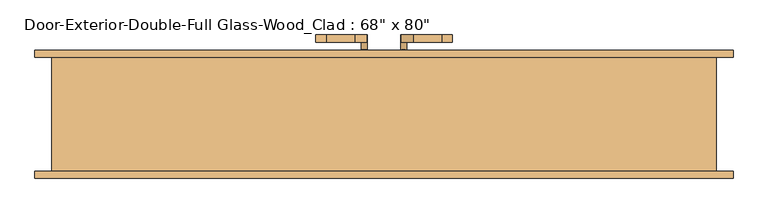
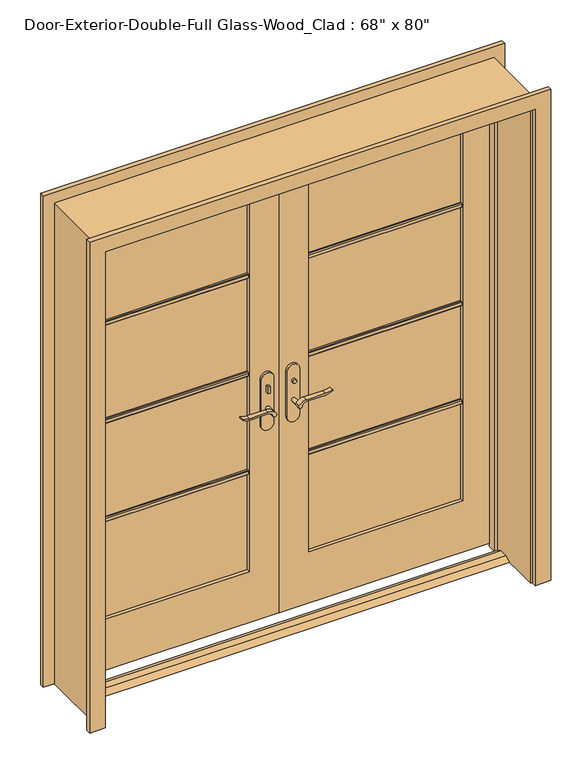
"""IFC4 building model written with IfcOpenShell, lengths in millimetres: door geometry."""

import ifcopenshell
import ifcopenshell.guid

model = None  # the IFC model being written
_history = None  # IfcOwnerHistory: only IFC2X3 demands one
_inside = {}  # id of a spatial element -> (the spatial element, [elements in it])
_under = {}  # id of a project, library or spatial element -> (it, [spatial elements below it])
_declared = {}  # id of a project -> (the project, [libraries it declares])
_typed = {}  # id of a type object -> (the type object, [elements of that type])
_made_of = {}  # id of a material, layer set ... -> (it, [elements and type objects made of it])


def new_model(schema):
    """Start an empty IFC model of exactly this schema.

    Asked for "IFC4X3", IfcOpenShell would pick the latest addendum, in which some entities
    have other attributes; the version numbers below select the first issue.
    IFC2X3 requires an IfcOwnerHistory on every rooted entity: one is made here for all.
    """
    global model, _history
    if schema == "IFC4X3":
        model = ifcopenshell.file(schema_version=(4, 3, 0, 0))
    else:
        model = ifcopenshell.file(schema=schema)
    _inside.clear()
    _under.clear()
    _declared.clear()
    _typed.clear()
    _made_of.clear()
    _history = None
    if model.schema == "IFC2X3":
        org = make("IfcOrganization", Name="unknown")
        user = make(
            "IfcPersonAndOrganization",
            ThePerson=make("IfcPerson", FamilyName="unknown"),
            TheOrganization=org,
        )
        app = make(
            "IfcApplication",
            ApplicationDeveloper=org,
            Version="unknown",
            ApplicationFullName="unknown",
            ApplicationIdentifier="unknown",
        )
        _history = make(
            "IfcOwnerHistory",
            OwningUser=user,
            OwningApplication=app,
            ChangeAction="ADDED",
            CreationDate=0,
        )
    return model


def make(cls, **values):
    """One entity of the class cls with the attributes given. An attribute that is None is left unset."""
    return model.create_entity(
        cls, **{name: value for name, value in values.items() if value is not None}
    )


def rooted(cls, **values):
    """An entity with a GlobalId (a new one), such as an element, a storey or a relation."""
    return make(cls, GlobalId=ifcopenshell.guid.new(), OwnerHistory=_history, **values)


def si_unit(unit_type, name, prefix=None):
    """IfcSIUnit, for example si_unit("LENGTHUNIT", "METRE", prefix="MILLI")."""
    return make("IfcSIUnit", UnitType=unit_type, Prefix=prefix, Name=name)


def assignment(units):
    """IfcUnitAssignment: the units of a project."""
    return None if units is None else make("IfcUnitAssignment", Units=units)


def point(xyz):
    """IfcCartesianPoint."""
    return None if xyz is None else make("IfcCartesianPoint", Coordinates=xyz)


def direction(xyz):
    """IfcDirection."""
    return None if xyz is None else make("IfcDirection", DirectionRatios=xyz)


def frame(location, z_axis=None, x_axis=None):
    """IfcAxis2Placement3D, a coordinate frame: its origin and axes. An axis left out is left unset."""
    return make(
        "IfcAxis2Placement3D",
        Location=point(location),
        Axis=direction(z_axis),
        RefDirection=direction(x_axis),
    )


def frame_2d(location, x_axis=None):
    """IfcAxis2Placement2D, a coordinate frame in the plane: its origin and x axis."""
    return make(
        "IfcAxis2Placement2D", Location=point(location), RefDirection=direction(x_axis)
    )


def origin():
    """The frame at (0, 0, 0) with its axes left unset."""
    return frame((0.0, 0.0, 0.0))


def place(relative_to, where):
    """IfcLocalPlacement: puts the frame where relative to a parent placement (None: the world)."""
    return make(
        "IfcLocalPlacement", PlacementRelTo=relative_to, RelativePlacement=where
    )


def context(
    kind, dimensions, precision=None, world=None, true_north=None, identifier=None
):
    """IfcGeometricRepresentationContext, for example the 3D "Model" context."""
    return make(
        "IfcGeometricRepresentationContext",
        ContextIdentifier=identifier,
        ContextType=kind,
        CoordinateSpaceDimension=dimensions,
        Precision=precision,
        WorldCoordinateSystem=world,
        TrueNorth=true_north,
    )


def project(units=None, contexts=None):
    """IfcProject with its units and contexts."""
    return rooted(
        "IfcProject",
        Name="project",
        RepresentationContexts=contexts,
        UnitsInContext=assignment(units),
    )


def spatial(cls, under=None, at=None, **own):
    """A site, building, storey or space (cls), placed at a placement, below another one or the project."""
    s = rooted(cls, ObjectPlacement=at, **own)
    if under is not None:
        _under.setdefault(under.id(), (under, []))[1].append(s)
    return s


def polyline(points):
    """IfcPolyline through the points."""
    return make("IfcPolyline", Points=[point(p) for p in points])


def circle_curve(where, radius):
    """IfcCircle in the frame where."""
    return make("IfcCircle", Position=where, Radius=radius)


def trimmed(basis, trim1, trim2, sense, master):
    """IfcTrimmedCurve: the piece of a basis curve between two trims."""
    return make(
        "IfcTrimmedCurve",
        BasisCurve=basis,
        Trim1=trim1,
        Trim2=trim2,
        SenseAgreement=sense,
        MasterRepresentation=master,
    )


def segment(curve, same_sense, transition):
    """IfcCompositeCurveSegment."""
    return make(
        "IfcCompositeCurveSegment",
        Transition=transition,
        SameSense=same_sense,
        ParentCurve=curve,
    )


def composite_curve(segments, self_intersect=None):
    """IfcCompositeCurve: segments joined end to end."""
    return make("IfcCompositeCurve", Segments=segments, SelfIntersect=self_intersect)


def outline(outer, holes=None, kind="AREA"):
    """IfcArbitraryClosedProfileDef: a profile drawn as a closed curve; with holes, ...WithVoids."""
    if holes is None:
        return make("IfcArbitraryClosedProfileDef", ProfileType=kind, OuterCurve=outer)
    return make(
        "IfcArbitraryProfileDefWithVoids",
        ProfileType=kind,
        OuterCurve=outer,
        InnerCurves=holes,
    )


def extrude(swept, where, along, depth):
    """IfcExtrudedAreaSolid: the profile swept, set in the frame where, extruded along a direction by depth."""
    return make(
        "IfcExtrudedAreaSolid",
        SweptArea=swept,
        Position=where,
        ExtrudedDirection=direction(along),
        Depth=depth,
    )


def faces_of(points, faces, orient=None, outer=None):
    """IfcFace entities. A face is a list of loops; a loop is a list of indices into points, from 0.

    orient and outer hold one flag for each loop. By default every Orientation is true, the
    first loop of a face is its IfcFaceOuterBound and the others are IfcFaceBound.
    """
    made = []
    for i, loops in enumerate(faces):
        bounds = []
        for j, loop in enumerate(loops):
            is_outer = j == 0 if outer is None else outer[i][j]
            bounds.append(
                make(
                    "IfcFaceOuterBound" if is_outer else "IfcFaceBound",
                    Bound=make("IfcPolyLoop", Polygon=[points[k] for k in loop]),
                    Orientation=True if orient is None else orient[i][j],
                )
            )
        made.append(make("IfcFace", Bounds=bounds))
    return made


def faceted_brep(points, faces, orient=None, outer=None, voids=None):
    """IfcFacetedBrep: a solid bounded by flat faces; with voids (closed shells), ...WithVoids."""
    shared = [point(p) for p in points]
    hull = make("IfcClosedShell", CfsFaces=faces_of(shared, faces, orient, outer))
    if voids is None:
        return make("IfcFacetedBrep", Outer=hull)
    return make(
        "IfcFacetedBrepWithVoids",
        Outer=hull,
        Voids=[
            make(cls, CfsFaces=faces_of(shared, fs, o, b)) for cls, fs, o, b in voids
        ],
    )


def shape(context_of_items, identifier, shape_type, items):
    """IfcShapeRepresentation: the items that make up one representation, for example the "Body"."""
    return make(
        "IfcShapeRepresentation",
        ContextOfItems=context_of_items,
        RepresentationIdentifier=identifier,
        RepresentationType=shape_type,
        Items=items,
    )


def source(mapping_origin, context_of_items, identifier, shape_type, items):
    """IfcRepresentationMap: a shape defined once, which mapped items show again and again."""
    return make(
        "IfcRepresentationMap",
        MappingOrigin=mapping_origin,
        MappedRepresentation=shape(context_of_items, identifier, shape_type, items),
    )


def transform(
    local_origin,
    x_axis=None,
    y_axis=None,
    z_axis=None,
    scale=None,
    scale2=None,
    scale3=None,
    uniform=True,
):
    """IfcCartesianTransformationOperator3D, or its non-uniform kind. x_axis, y_axis, z_axis: its Axis1, 2, 3."""
    if uniform:
        return make(
            "IfcCartesianTransformationOperator3D",
            Axis1=direction(x_axis),
            Axis2=direction(y_axis),
            LocalOrigin=point(local_origin),
            Scale=scale,
            Axis3=direction(z_axis),
        )
    return make(
        "IfcCartesianTransformationOperator3DnonUniform",
        Axis1=direction(x_axis),
        Axis2=direction(y_axis),
        LocalOrigin=point(local_origin),
        Scale=scale,
        Axis3=direction(z_axis),
        Scale2=scale2,
        Scale3=scale3,
    )


def mapped(mapping_source, mapping_target):
    """IfcMappedItem: shows the shape of a source again, moved by a transform."""
    return make(
        "IfcMappedItem", MappingSource=mapping_source, MappingTarget=mapping_target
    )


def made_of(thing, what):
    """Note that an element or type object is made of a material, layer set ...; save() writes the relation."""
    if what is not None:
        _made_of.setdefault(what.id(), (what, []))[1].append(thing)
    return thing


def element(
    cls,
    number,
    at=None,
    inside=None,
    cuts=None,
    type_object=None,
    material=None,
    context=None,
    identifier="Body",
    shape_type=None,
    held_by="IfcProductDefinitionShape",
    body=None,
    shapes=None,
    **own,
):
    """One element of the class cls, such as IfcWall. Its Tag is "e" and its number.

    at: its placement. inside: the storey or other place that contains it. cuts: it is an
    opening in that element (IfcRelVoidsElement). A single representation is given by context,
    identifier, shape_type and body (its items); several are given by shapes. held_by: the class
    of the entity that holds the representations. save() writes the other relations.
    """
    e = rooted(cls, Tag="e%d" % number, ObjectPlacement=at, **own)
    if body is not None:
        shapes = [shape(context, identifier, shape_type, body)]
    if shapes is not None:
        e.Representation = make(held_by, Representations=shapes)
    if inside is not None:
        _inside.setdefault(inside.id(), (inside, []))[1].append(e)
    if cuts is not None:
        rooted(
            "IfcRelVoidsElement", RelatingBuildingElement=cuts, RelatedOpeningElement=e
        )
    if type_object is not None:
        _typed.setdefault(type_object.id(), (type_object, []))[1].append(e)
    return made_of(e, material)


def aggregate(whole, parts):
    """IfcRelAggregates: a whole, such as a stair, and the parts it consists of."""
    return rooted("IfcRelAggregates", RelatingObject=whole, RelatedObjects=parts)


def save(model, path):
    """Write the relations noted so far, then the file.

    IfcRelAggregates (storeys below a building ...), IfcRelContainedInSpatialStructure (elements
    in a storey), IfcRelDefinesByType, IfcRelAssociatesMaterial and IfcRelDeclares: one each for
    every whole, place, type object, material and project.
    """
    for whole, parts in _under.values():
        aggregate(whole, parts)
    for where, things in _inside.values():
        rooted(
            "IfcRelContainedInSpatialStructure",
            RelatedElements=things,
            RelatingStructure=where,
        )
    for kind, things in _typed.values():
        rooted("IfcRelDefinesByType", RelatedObjects=things, RelatingType=kind)
    for what, things in _made_of.values():
        rooted("IfcRelAssociatesMaterial", RelatedObjects=things, RelatingMaterial=what)
    for by, libraries in _declared.values():
        rooted("IfcRelDeclares", RelatingContext=by, RelatedDefinitions=libraries)
    model.write(path)


def door_f3362da7(model_context):
    return source(origin(), model_context, "Body", "SolidModel", [
        extrude(outline(polyline([(19.05, 12.7), (53.975, 12.7), (79.375, 0.0), (-6.35, 0.0), (19.05, 12.7)])), frame((-863.6, 0.0, 0.0), z_axis=(1.0, 0.0, 0.0), x_axis=(0.0, 1.0, 0.0)), (0.0, 0.0, 1.0), 1727.2),
        extrude(outline(polyline([(-47.4019111, 94.3), (-57.4019111, 94.3), (-57.4019111, 104.3), (-47.4019111, 104.3), (-47.4019111, 94.3)])), frame((0.0, 0.0, 981.9), z_axis=(0.0, 0.0, 1.0), x_axis=(1.0, 0.0, 0.0)), (0.0, 0.0, 1.0), 30.0),
        extrude(outline(composite_curve([segment(trimmed(circle_curve(frame_2d((996.9, -52.4019111)), 8.0), [point((996.9, -60.4019111))], [point((996.9, -44.4019111))], False, "CARTESIAN"), True, "CONTINUOUS"), segment(trimmed(circle_curve(frame_2d((996.9, -52.4019111)), 8.0), [point((996.9, -44.4019111))], [point((996.9, -60.4019111))], False, "CARTESIAN"), True, "CONTINUOUS")], self_intersect=False)), frame((0.0, 159.225, 0.0), z_axis=(0.0, 1.0, 0.0), x_axis=(0.0, 0.0, 1.0)), (0.0, 0.0, 1.0), 10.0),
        extrude(outline(composite_curve([segment(trimmed(circle_curve(frame_2d((897.1555521, -76.0694241)), 37.2832219), [point((919.0523287, -45.8937749))], [point((934.4, -77.7693445))], False, "CARTESIAN"), True, "CONTINUOUS"), segment(polyline([(934.4, -77.7693445), (934.4, -154.045502)]), True, "CONTINUOUS"), segment(trimmed(circle_curve(frame_2d((1017.6850638, -153.9791202)), 83.2850902), [point((934.4, -154.045502))], [point((939.4, -182.4019111))], True, "CARTESIAN"), True, "CONTINUOUS"), segment(polyline([(939.4, -182.4019111), (936.6135558, -182.4019111)]), True, "CONTINUOUS"), segment(trimmed(circle_curve(frame_2d((986.6709207, -150.4622499)), 59.3791355), [point((936.6135558, -182.4019111))], [point((927.4, -154.045502))], False, "CARTESIAN"), True, "CONTINUOUS"), segment(polyline([(927.4, -154.045502), (927.4, -77.7881013)]), True, "CONTINUOUS"), segment(trimmed(circle_curve(frame_2d((909.2738613, -77.7881013)), 18.1261387), [point((927.4, -77.7881013))], [point((914.4, -60.4019111))], True, "CARTESIAN"), True, "CONTINUOUS"), segment(trimmed(circle_curve(frame_2d((914.4, -52.4019111)), 8.0), [point((914.4, -60.4019111))], [point((919.0523287, -45.8937749))], False, "CARTESIAN"), True, "CONTINUOUS")], self_intersect=False)), frame((0.0, 54.3, 0.0), z_axis=(0.0, 1.0, 0.0), x_axis=(0.0, 0.0, 1.0)), (0.0, 0.0, 1.0), 20.0),
        extrude(outline(composite_curve([segment(trimmed(circle_curve(frame_2d((914.4, -52.4019111)), 8.0), [point((914.3999903, -60.4019111))], [point((919.0523287, -45.8937749))], False, "CARTESIAN"), True, "CONTINUOUS"), segment(trimmed(circle_curve(frame_2d((897.1555521, -76.0694241)), 37.2832219), [point((919.0523287, -45.8937749))], [point((934.4, -77.7693445))], False, "CARTESIAN"), True, "CONTINUOUS"), segment(polyline([(934.4, -77.7693445), (934.4, -154.045502)]), True, "CONTINUOUS"), segment(trimmed(circle_curve(frame_2d((1017.6850638, -153.9791202)), 83.2850902), [point((934.4, -154.045502))], [point((939.4, -182.4019111))], True, "CARTESIAN"), True, "CONTINUOUS"), segment(polyline([(939.4, -182.4019111), (936.6135558, -182.4019111)]), True, "CONTINUOUS"), segment(trimmed(circle_curve(frame_2d((986.6709207, -150.4622499)), 59.3791355), [point((936.6135558, -182.4019111))], [point((927.4, -154.045502))], False, "CARTESIAN"), True, "CONTINUOUS"), segment(polyline([(927.4, -154.045502), (927.4, -77.788099)]), True, "CONTINUOUS"), segment(trimmed(circle_curve(frame_2d((909.2738682, -77.788099)), 18.1261318), [point((927.4, -77.788099))], [point((914.3999903, -60.4019111))], True, "CARTESIAN"), True, "CONTINUOUS")], self_intersect=False)), frame((0.0, 189.225, 0.0), z_axis=(0.0, 1.0, 0.0), x_axis=(0.0, 0.0, 1.0)), (0.0, 0.0, 1.0), 20.0),
        extrude(outline(composite_curve([segment(trimmed(circle_curve(frame_2d((914.4, -52.4019111)), 8.0), [point((914.4, -60.4019111))], [point((914.4, -44.4019111))], False, "CARTESIAN"), True, "CONTINUOUS"), segment(trimmed(circle_curve(frame_2d((914.4, -52.4019111)), 8.0), [point((914.4, -44.4019111))], [point((914.4, -60.4019111))], False, "CARTESIAN"), True, "CONTINUOUS")], self_intersect=False)), frame((0.0, 74.3, 0.0), z_axis=(0.0, 1.0, 0.0), x_axis=(0.0, 0.0, 1.0)), (0.0, 0.0, 1.0), 30.0),
        extrude(outline(composite_curve([segment(trimmed(circle_curve(frame_2d((914.4, -52.4019111)), 8.0), [point((914.4, -60.4019111))], [point((914.4, -44.4019111))], False, "CARTESIAN"), True, "CONTINUOUS"), segment(trimmed(circle_curve(frame_2d((914.4, -52.4019111)), 8.0), [point((914.4, -44.4019111))], [point((914.4, -60.4019111))], False, "CARTESIAN"), True, "CONTINUOUS")], self_intersect=False)), frame((0.0, 159.225, 0.0), z_axis=(0.0, 1.0, 0.0), x_axis=(0.0, 0.0, 1.0)), (0.0, 0.0, 1.0), 30.0),
        extrude(outline(composite_curve([segment(polyline([(844.4, -27.4019111), (1039.4, -27.4019111)]), True, "CONTINUOUS"), segment(trimmed(circle_curve(frame_2d((1039.4, -52.4019111)), 25.0), [point((1039.4, -27.4019111))], [point((1039.4, -77.4019111))], False, "CARTESIAN"), True, "CONTINUOUS"), segment(polyline([(1039.4, -77.4019111), (844.4, -77.4019111)]), True, "CONTINUOUS"), segment(trimmed(circle_curve(frame_2d((844.4, -52.4019111)), 25.0), [point((844.4, -77.4019111))], [point((844.4, -27.4019111))], False, "CARTESIAN"), True, "CONTINUOUS")], self_intersect=False)), frame((0.0, 104.3, 0.0), z_axis=(0.0, 1.0, 0.0), x_axis=(0.0, 0.0, 1.0)), (0.0, 0.0, 1.0), 10.0),
        extrude(outline(composite_curve([segment(polyline([(844.4, -27.4019111), (1039.4, -27.4019111)]), True, "CONTINUOUS"), segment(trimmed(circle_curve(frame_2d((1039.4, -52.4019111)), 25.0), [point((1039.4, -27.4019111))], [point((1039.4, -77.4019111))], False, "CARTESIAN"), True, "CONTINUOUS"), segment(polyline([(1039.4, -77.4019111), (844.4, -77.4019111)]), True, "CONTINUOUS"), segment(trimmed(circle_curve(frame_2d((844.4, -52.4019111)), 25.0), [point((844.4, -77.4019111))], [point((844.4, -27.4019111))], False, "CARTESIAN"), True, "CONTINUOUS")], self_intersect=False)), frame((0.0, 149.225, 0.0), z_axis=(0.0, 1.0, 0.0), x_axis=(0.0, 0.0, 1.0)), (0.0, 0.0, 1.0), 10.0),
        extrude(outline(polyline([(47.3875, 169.225), (57.3875, 169.225), (57.3875, 159.225), (47.3875, 159.225), (47.3875, 169.225)])), frame((0.0, 0.0, 981.9), z_axis=(0.0, 0.0, 1.0), x_axis=(1.0, 0.0, 0.0)), (0.0, 0.0, 1.0), 30.0),
        extrude(outline(composite_curve([segment(trimmed(circle_curve(frame_2d((996.9, 52.3875)), 8.0), [point((996.9, 60.3875))], [point((996.9, 44.3875))], False, "CARTESIAN"), True, "CONTINUOUS"), segment(trimmed(circle_curve(frame_2d((996.9, 52.3875)), 8.0), [point((996.9, 44.3875))], [point((996.9, 60.3875))], False, "CARTESIAN"), True, "CONTINUOUS")], self_intersect=False)), frame((0.0, 94.3, 0.0), z_axis=(0.0, 1.0, 0.0), x_axis=(0.0, 0.0, 1.0)), (0.0, 0.0, 1.0), 10.0),
        extrude(outline(composite_curve([segment(trimmed(circle_curve(frame_2d((914.4, 52.3875)), 8.0), [point((919.0523287, 45.8793637))], [point((914.4, 60.3875))], False, "CARTESIAN"), True, "CONTINUOUS"), segment(trimmed(circle_curve(frame_2d((909.2738613, 77.7736901)), 18.1261387), [point((914.4, 60.3875))], [point((927.4, 77.7736901))], True, "CARTESIAN"), True, "CONTINUOUS"), segment(polyline([(927.4, 77.7736901), (927.4, 154.0310909)]), True, "CONTINUOUS"), segment(trimmed(circle_curve(frame_2d((986.6709207, 150.4478388)), 59.3791355), [point((927.4, 154.0310909))], [point((936.6135558, 182.3875))], False, "CARTESIAN"), True, "CONTINUOUS"), segment(polyline([(936.6135558, 182.3875), (939.4, 182.3875)]), True, "CONTINUOUS"), segment(trimmed(circle_curve(frame_2d((1017.6850638, 153.9647091)), 83.2850902), [point((939.4, 182.3875))], [point((934.4, 154.0310909))], True, "CARTESIAN"), True, "CONTINUOUS"), segment(polyline([(934.4, 154.0310909), (934.4, 77.7549333)]), True, "CONTINUOUS"), segment(trimmed(circle_curve(frame_2d((897.1555521, 76.0550129)), 37.2832219), [point((934.4, 77.7549333))], [point((919.0523287, 45.8793637))], False, "CARTESIAN"), True, "CONTINUOUS")], self_intersect=False)), frame((0.0, 189.225, 0.0), z_axis=(0.0, 1.0, 0.0), x_axis=(0.0, 0.0, 1.0)), (0.0, 0.0, 1.0), 20.0),
        extrude(outline(composite_curve([segment(trimmed(circle_curve(frame_2d((909.2738682, 77.7736878)), 18.1261318), [point((914.3999903, 60.3875))], [point((927.4, 77.7736878))], True, "CARTESIAN"), True, "CONTINUOUS"), segment(polyline([(927.4, 77.7736878), (927.4, 154.0310909)]), True, "CONTINUOUS"), segment(trimmed(circle_curve(frame_2d((986.6709207, 150.4478388)), 59.3791355), [point((927.4, 154.0310909))], [point((936.6135558, 182.3875))], False, "CARTESIAN"), True, "CONTINUOUS"), segment(polyline([(936.6135558, 182.3875), (939.4, 182.3875)]), True, "CONTINUOUS"), segment(trimmed(circle_curve(frame_2d((1017.6850638, 153.9647091)), 83.2850902), [point((939.4, 182.3875))], [point((934.4, 154.0310909))], True, "CARTESIAN"), True, "CONTINUOUS"), segment(polyline([(934.4, 154.0310909), (934.4, 77.7549333)]), True, "CONTINUOUS"), segment(trimmed(circle_curve(frame_2d((897.1555521, 76.0550129)), 37.2832219), [point((934.4, 77.7549333))], [point((919.0523287, 45.8793637))], False, "CARTESIAN"), True, "CONTINUOUS"), segment(trimmed(circle_curve(frame_2d((914.4, 52.3875)), 8.0), [point((919.0523287, 45.8793637))], [point((914.3999903, 60.3875))], False, "CARTESIAN"), True, "CONTINUOUS")], self_intersect=False)), frame((0.0, 54.3, 0.0), z_axis=(0.0, 1.0, 0.0), x_axis=(0.0, 0.0, 1.0)), (0.0, 0.0, 1.0), 20.0),
        extrude(outline(composite_curve([segment(trimmed(circle_curve(frame_2d((914.4, 52.3875)), 8.0), [point((914.4, 60.3875))], [point((914.4, 44.3875))], False, "CARTESIAN"), True, "CONTINUOUS"), segment(trimmed(circle_curve(frame_2d((914.4, 52.3875)), 8.0), [point((914.4, 44.3875))], [point((914.4, 60.3875))], False, "CARTESIAN"), True, "CONTINUOUS")], self_intersect=False)), frame((0.0, 159.225, 0.0), z_axis=(0.0, 1.0, 0.0), x_axis=(0.0, 0.0, 1.0)), (0.0, 0.0, 1.0), 30.0),
        extrude(outline(composite_curve([segment(trimmed(circle_curve(frame_2d((914.4, 52.3875)), 8.0), [point((914.4, 60.3875))], [point((914.4, 44.3875))], False, "CARTESIAN"), True, "CONTINUOUS"), segment(trimmed(circle_curve(frame_2d((914.4, 52.3875)), 8.0), [point((914.4, 44.3875))], [point((914.4, 60.3875))], False, "CARTESIAN"), True, "CONTINUOUS")], self_intersect=False)), frame((0.0, 74.3, 0.0), z_axis=(0.0, 1.0, 0.0), x_axis=(0.0, 0.0, 1.0)), (0.0, 0.0, 1.0), 30.0),
        extrude(outline(composite_curve([segment(trimmed(circle_curve(frame_2d((844.4, 52.3875)), 25.0), [point((844.4, 27.3875))], [point((844.4, 77.3875))], False, "CARTESIAN"), True, "CONTINUOUS"), segment(polyline([(844.4, 77.3875), (1039.4, 77.3875)]), True, "CONTINUOUS"), segment(trimmed(circle_curve(frame_2d((1039.4, 52.3875)), 25.0), [point((1039.4, 77.3875))], [point((1039.4, 27.3875))], False, "CARTESIAN"), True, "CONTINUOUS"), segment(polyline([(1039.4, 27.3875), (844.4, 27.3875)]), True, "CONTINUOUS")], self_intersect=False)), frame((0.0, 149.225, 0.0), z_axis=(0.0, 1.0, 0.0), x_axis=(0.0, 0.0, 1.0)), (0.0, 0.0, 1.0), 10.0),
        extrude(outline(composite_curve([segment(trimmed(circle_curve(frame_2d((844.4, 52.3875)), 25.0), [point((844.4, 27.3875))], [point((844.4, 77.3875))], False, "CARTESIAN"), True, "CONTINUOUS"), segment(polyline([(844.4, 77.3875), (1039.4, 77.3875)]), True, "CONTINUOUS"), segment(trimmed(circle_curve(frame_2d((1039.4, 52.3875)), 25.0), [point((1039.4, 77.3875))], [point((1039.4, 27.3875))], False, "CARTESIAN"), True, "CONTINUOUS"), segment(polyline([(1039.4, 27.3875), (844.4, 27.3875)]), True, "CONTINUOUS")], self_intersect=False)), frame((0.0, 104.3, 0.0), z_axis=(0.0, 1.0, 0.0), x_axis=(0.0, 0.0, 1.0)), (0.0, 0.0, 1.0), 10.0),
        extrude(outline(polyline([(128.27, 1502.171875), (128.27, 1483.121875), (121.92, 1483.121875), (118.745, 1486.296875), (118.745, 1498.996875), (121.92, 1502.171875), (128.27, 1502.171875)])), frame((120.65, 0.0, 0.0), z_axis=(1.0, 0.0, 0.0), x_axis=(0.0, 1.0, 0.0)), (0.0, 0.0, 1.0), 622.3),
        extrude(outline(polyline([(128.27, 1081.88125), (128.27, 1062.83125), (121.92, 1062.83125), (118.745, 1066.00625), (118.745, 1078.70625), (121.92, 1081.88125), (128.27, 1081.88125)])), frame((120.65, 0.0, 0.0), z_axis=(1.0, 0.0, 0.0), x_axis=(0.0, 1.0, 0.0)), (0.0, 0.0, 1.0), 622.3),
        extrude(outline(polyline([(128.27, 661.590625), (128.27, 642.540625), (121.92, 642.540625), (118.745, 645.715625), (118.745, 658.415625), (121.92, 661.590625), (128.27, 661.590625)])), frame((120.65, 0.0, 0.0), z_axis=(1.0, 0.0, 0.0), x_axis=(0.0, 1.0, 0.0)), (0.0, 0.0, 1.0), 622.3),
        extrude(outline(polyline([(135.255, 1502.171875), (141.605, 1502.171875), (144.78, 1498.996875), (144.78, 1486.296875), (141.605, 1483.121875), (135.255, 1483.121875), (135.255, 1502.171875)])), frame((-742.95, 0.0, 0.0), z_axis=(1.0, 0.0, 0.0), x_axis=(0.0, 1.0, 0.0)), (0.0, 0.0, 1.0), 622.3),
        extrude(outline(polyline([(135.255, 1081.88125), (141.605, 1081.88125), (144.78, 1078.70625), (144.78, 1066.00625), (141.605, 1062.83125), (135.255, 1062.83125), (135.255, 1081.88125)])), frame((-742.95, 0.0, 0.0), z_axis=(1.0, 0.0, 0.0), x_axis=(0.0, 1.0, 0.0)), (0.0, 0.0, 1.0), 622.3),
        extrude(outline(polyline([(135.255, 661.590625), (141.605, 661.590625), (144.78, 658.415625), (144.78, 645.715625), (141.605, 642.540625), (135.255, 642.540625), (135.255, 661.590625)])), frame((-742.95, 0.0, 0.0), z_axis=(1.0, 0.0, 0.0), x_axis=(0.0, 1.0, 0.0)), (0.0, 0.0, 1.0), 622.3),
        extrude(outline(polyline([(135.255, 1502.171875), (141.605, 1502.171875), (144.78, 1498.996875), (144.78, 1486.296875), (141.605, 1483.121875), (135.255, 1483.121875), (135.255, 1502.171875)])), frame((120.65, 0.0, 0.0), z_axis=(1.0, 0.0, 0.0), x_axis=(0.0, 1.0, 0.0)), (0.0, 0.0, 1.0), 622.3),
        extrude(outline(polyline([(135.255, 1081.88125), (141.605, 1081.88125), (144.78, 1078.70625), (144.78, 1066.00625), (141.605, 1062.83125), (135.255, 1062.83125), (135.255, 1081.88125)])), frame((120.65, 0.0, 0.0), z_axis=(1.0, 0.0, 0.0), x_axis=(0.0, 1.0, 0.0)), (0.0, 0.0, 1.0), 622.3),
        extrude(outline(polyline([(135.255, 661.590625), (141.605, 661.590625), (144.78, 658.415625), (144.78, 645.715625), (141.605, 642.540625), (135.255, 642.540625), (135.255, 661.590625)])), frame((120.65, 0.0, 0.0), z_axis=(1.0, 0.0, 0.0), x_axis=(0.0, 1.0, 0.0)), (0.0, 0.0, 1.0), 622.3),
        extrude(outline(polyline([(128.27, 1502.171875), (128.27, 1483.121875), (121.92, 1483.121875), (118.745, 1486.296875), (118.745, 1498.996875), (121.92, 1502.171875), (128.27, 1502.171875)])), frame((-742.95, 0.0, 0.0), z_axis=(1.0, 0.0, 0.0), x_axis=(0.0, 1.0, 0.0)), (0.0, 0.0, 1.0), 622.3),
        extrude(outline(polyline([(128.27, 1081.88125), (128.27, 1062.83125), (121.92, 1062.83125), (118.745, 1066.00625), (118.745, 1078.70625), (121.92, 1081.88125), (128.27, 1081.88125)])), frame((-742.95, 0.0, 0.0), z_axis=(1.0, 0.0, 0.0), x_axis=(0.0, 1.0, 0.0)), (0.0, 0.0, 1.0), 622.3),
        extrude(outline(polyline([(128.27, 661.590625), (128.27, 642.540625), (121.92, 642.540625), (118.745, 645.715625), (118.745, 658.415625), (121.92, 661.590625), (128.27, 661.590625)])), frame((-742.95, 0.0, 0.0), z_axis=(1.0, 0.0, 0.0), x_axis=(0.0, 1.0, 0.0)), (0.0, 0.0, 1.0), 622.3),
        extrude(outline(polyline([(0.0, 869.95), (0.0, 933.45), (2101.85, 933.45), (2101.85, -933.45), (0.0, -933.45), (0.0, -869.95), (2038.35, -869.95), (2038.35, 869.95), (0.0, 869.95)])), frame((0.0, 149.225, 0.0), z_axis=(0.0, 1.0, 0.0), x_axis=(0.0, 0.0, 1.0)), (0.0, 0.0, 1.0), 19.05),
        extrude(outline(polyline([(0.0, 869.95), (0.0, 933.45), (2101.85, 933.45), (2101.85, -933.45), (0.0, -933.45), (0.0, -869.95), (2038.35, -869.95), (2038.35, 869.95), (0.0, 869.95)])), frame((0.0, -174.625, 0.0), z_axis=(0.0, 1.0, 0.0), x_axis=(0.0, 0.0, 1.0)), (0.0, 0.0, 1.0), 19.05),
        extrude(outline(polyline([(12.7, 863.6), (2032.0, 863.6), (2032.0, 1.5875), (12.7, 1.5875), (12.7, 863.6)]), holes=[polyline([(1912.9375, 120.65), (1912.9375, 742.95), (231.775, 742.95), (231.775, 120.65), (1912.9375, 120.65)])]), frame((0.0, 114.3, 0.0), z_axis=(0.0, 1.0, 0.0), x_axis=(0.0, 0.0, 1.0)), (0.0, 0.0, 1.0), 34.925),
        extrude(outline(polyline([(2032.0, -863.6), (12.7, -863.6), (12.7, -1.6019111), (2032.0, -1.6019111), (2032.0, -863.6)]), holes=[polyline([(231.775, -742.95), (1912.9375, -742.95), (1912.9375, -120.65), (231.775, -120.65), (231.775, -742.95)])]), frame((0.0, 114.3, 0.0), z_axis=(0.0, 1.0, 0.0), x_axis=(0.0, 0.0, 1.0)), (0.0, 0.0, 1.0), 34.925),
        faceted_brep([(889.0, 149.225, 0.0), (889.0, -155.575, 0.0), (863.6, -155.575, 0.0), (863.6, 79.375, 0.0), (850.9, 79.375, 0.0), (850.9, 114.3, 0.0), (863.6, 114.3, 0.0), (863.6, 149.225, 0.0), (889.0, 149.225, 2057.4), (889.0, -155.575, 2057.4), (-889.0, -155.575, 2057.4), (-889.0, -155.575, 0.0), (-863.6, -155.575, 0.0), (-863.6, -155.575, 2032.0), (863.6, -155.575, 2032.0), (863.6, 79.375, 2032.0), (-863.6, 79.375, 2032.0), (-863.6, 79.375, 0.0), (-850.9, 79.375, 0.0), (-850.9, 79.375, 2019.3), (850.9, 79.375, 2019.3), (850.9, 114.3, 2019.3), (1.5875, 114.3, 2019.3), (-1.6019111, 114.3, 2019.3), (-850.9, 114.3, 2019.3), (-850.9, 114.3, 0.0), (-863.6, 114.3, 0.0), (-863.6, 114.3, 2032.0), (-1.6019111, 114.3, 2032.0), (1.5875, 114.3, 2032.0), (863.6, 114.3, 2032.0), (863.6, 149.225, 2032.0), (1.5875, 149.225, 2032.0), (-1.6019111, 149.225, 2032.0), (-863.6, 149.225, 2032.0), (-863.6, 149.225, 0.0), (-889.0, 149.225, 0.0), (-889.0, 149.225, 2057.4)], [[[0, 1, 2, 3, 4, 5, 6, 7]], [[1, 0, 8, 9]], [[2, 1, 9, 10, 11, 12, 13, 14]], [[3, 2, 14, 15]], [[4, 3, 15, 16, 17, 18, 19, 20]], [[5, 4, 20, 21]], [[6, 5, 21, 22, 23, 24, 25, 26, 27, 28, 29, 30]], [[7, 6, 30, 31]], [[0, 7, 31, 32, 33, 34, 35, 36, 37, 8]], [[9, 8, 37, 10]], [[14, 13, 16, 15]], [[20, 19, 24, 23, 22, 21]], [[31, 30, 29, 28, 27, 34, 33, 32]], [[12, 11, 36, 35, 26, 25, 18, 17]], [[11, 10, 37, 36]], [[13, 12, 17, 16]], [[19, 18, 25, 24]], [[27, 26, 35, 34]]]),
        extrude(outline(polyline([(742.95, 128.27), (120.65, 128.27), (120.65, 135.255), (742.95, 135.255), (742.95, 128.27)])), frame((0.0, 0.0, 231.775), z_axis=(0.0, 0.0, 1.0), x_axis=(1.0, 0.0, 0.0)), (0.0, 0.0, 1.0), 1681.1625),
        extrude(outline(polyline([(-120.65, 128.27), (-742.95, 128.27), (-742.95, 135.255), (-120.65, 135.255), (-120.65, 128.27)])), frame((0.0, 0.0, 231.775), z_axis=(0.0, 0.0, 1.0), x_axis=(1.0, 0.0, 0.0)), (0.0, 0.0, 1.0), 1681.1625),
    ])


if __name__ == "__main__":
    model = new_model("IFC4")
    model_context = context("Model", 3, world=origin())
    ifc_project = project(units=[si_unit("LENGTHUNIT", "METRE", prefix="MILLI")], contexts=[model_context])
    site = spatial("IfcSite", under=ifc_project)
    building = spatial("IfcBuilding", under=site)
    placement = place(None, origin())
    door_shape = door_f3362da7(model_context)
    element("IfcDoor", 1, ObjectType="Door-Exterior-Double-Full Glass-Wood_Clad : 68\" x 80\"", at=placement, inside=building, context=model_context, shape_type="MappedRepresentation", body=[
        mapped(door_shape, transform((0.0, 0.0, 0.0), x_axis=(1.0, 0.0, 0.0), y_axis=(0.0, 1.0, 0.0), z_axis=(0.0, 0.0, 1.0))),
    ])
    save(model, "model.ifc")

# Revit data of these elements
# Type "Door-Exterior-Double-Full Glass-Wood_Clad : 68\" x 80\""
#   Type Mark = "21"
#   Assembly Code = "B2030100"
#   Analytic Construction = "French door, wood frame with double glass"
#   Top Rail = 0' - 4 11/16"
#   Threshold Offset [instance default] = 0' - 0 1/2"
#   Thickness = 0' - 1 3/8"
#   Thermal Resistance (R) = 1.9158 (h·ft²·°F)/BTU
#   Swing Angle [instance default] = 90.0000°
#   Stiles = 0' - 4 3/4"
#   Rough Width = 5' - 10"
#   Rough Height = 6' - 9"
#   Panel Width = 2' - 10"
#   Door Offset [instance default] = 0' - 0"
#   Height = 6' - 8"
#   Width = 5' - 8"
#   Heat Transfer Coefficient (U) = 0.5220 BTU/(h·ft²·°F)
#   Bottom Rail = 0' - 9 1/8"
#   Exterior Trim [instance default] = yes
#   Threshold [instance default] = yes
#   Show Grill [instance default] = yes
#   Function = 1
#   Trim Material = Cherry
#   Threshold Material = Cherry
#   Panel Material = Cherry
#   Glazing = Glass
#   Frame Material = Cherry
#   Door Handle Material = Aluminum
#   Visual Light Transmittance = 0
#   Solar Heat Gain Coefficient = 0
#   Wall Closure = (empty or 0)
#   Construction Type = (empty or 0)
# Element 1 (IfcDoor, "Door-Exterior-Double-Full Glass-Wood_Clad : 68\" x 80\"")
#   Materials on its faces: "Cherry", "Aluminum", "Glass"
# Materials
#   "Cherry": class "Wood", colour RGB 226 177 128, transparency 0, Description = "Prunus Serotina", Cost = 0
#   "Glass": class "Glass", colour RGB 0 128 192, transparency 0.75, Description = "Soda Lime Glass", Cost = 0
#   "Aluminum": class "Metal", colour RGB 247 247 247, transparency 0, Description = "Aluminum 6061", Cost = 0
